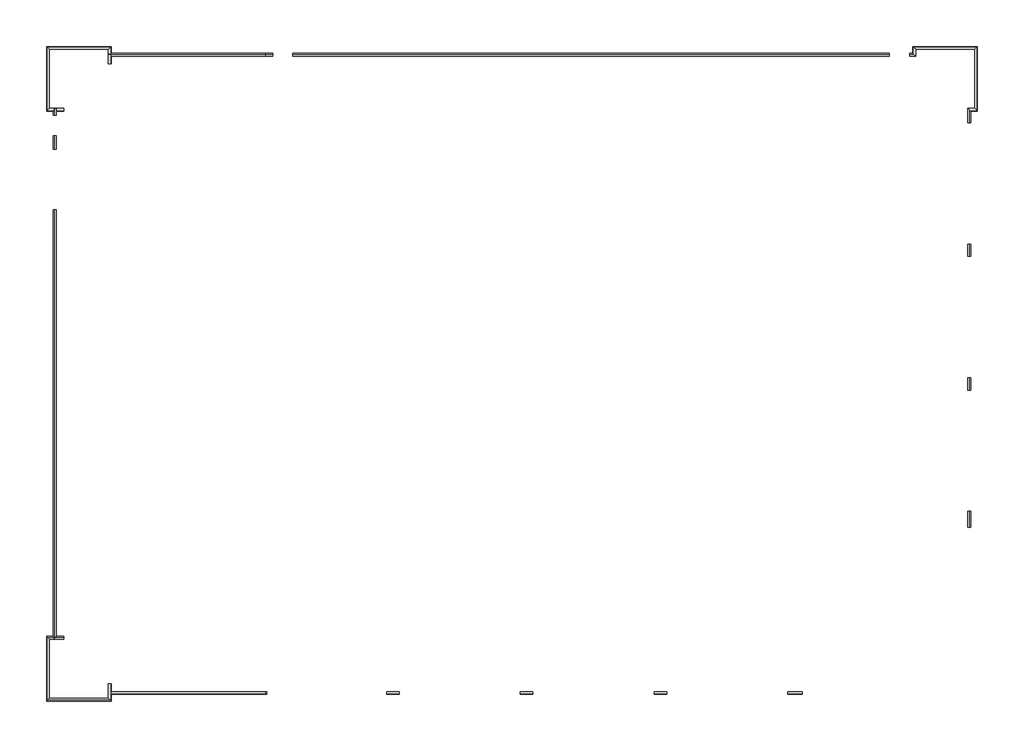
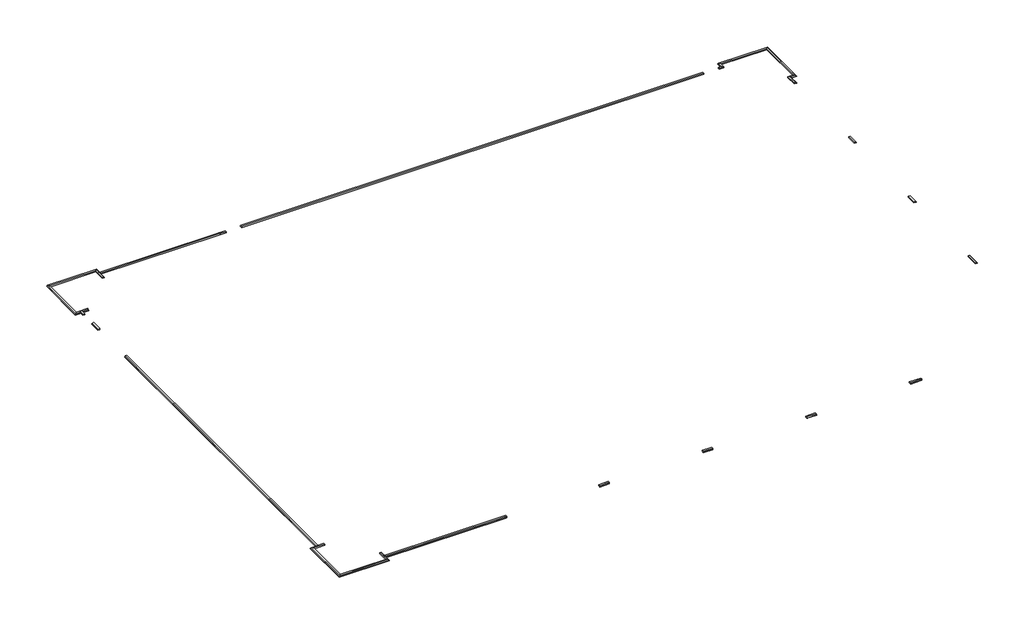
# One storey: 18 proxies.
"""IFC4 building model written with IfcOpenShell, lengths in millimetres."""

from ifc_helpers import new_model, si_unit, origin, place, context, project, spatial, faceted_brep, element, save

model = new_model("IFC4")

# Units and contexts
model_context = context("Model", 3, world=origin())
ifc_project = project(units=[si_unit("LENGTHUNIT", "METRE", prefix="MILLI")], contexts=[model_context])

# Site, building, storey
site = spatial("IfcSite", under=ifc_project)
building = spatial("IfcBuilding", under=site)
storey = spatial("IfcBuildingStorey", under=building, Name="CMU Watertable", Elevation=914.4)

# Proxies
placement = place(None, origin())
element("IfcBuildingElementProxy", 1, Name="Wall Sweeps", at=placement, inside=storey, context=model_context, shape_type="Brep", body=[
    faceted_brep([(-20031.8727721, 14336.3436943, 984.25), (-20031.8727721, 14428.4186943, 984.25), (-20031.8727721, 14463.3436943, 939.8), (-20031.8727721, 14463.3436943, 914.4), (-20031.8727721, 14447.4686943, 914.4), (-20031.8727721, 14336.3436943, 914.4), (-12953.2102721, 14336.3436943, 984.25), (-12953.2102721, 14336.3436943, 914.4), (-12953.2102721, 14345.8686943, 914.4), (-12953.2102721, 14447.4686943, 914.4), (-12953.2102721, 14463.3436943, 914.4), (-12953.2102721, 14463.3436943, 939.8), (-12953.2102721, 14428.4186943, 984.25)], [[[0, 1, 2, 3, 4, 5]], [[6, 7, 8, 9, 10, 11, 12]], [[1, 0, 6, 12]], [[2, 1, 12, 11]], [[3, 2, 11, 10]], [[5, 4, 3, 10, 9, 8, 7]], [[0, 5, 7, 6]]]),
])
element("IfcBuildingElementProxy", 2, Name="Wall Sweeps", at=placement, inside=storey, context=model_context, shape_type="Brep", body=[
    faceted_brep([(18820.6022279, 11967.7936943, 984.25), (18912.6772279, 11875.7186943, 984.25), (18947.6022279, 11840.7936943, 939.8), (18947.6022279, 11840.7936943, 914.4), (18820.6022279, 11967.7936943, 914.4), (18820.6022279, 11321.6811943, 984.25), (18820.6022279, 11321.6811943, 914.4), (18931.7272279, 11321.6811943, 914.4), (18947.6022279, 11321.6811943, 914.4), (18947.6022279, 11321.6811943, 939.8), (18912.6772279, 11321.6811943, 984.25)], [[[0, 1, 2, 3, 4]], [[5, 6, 7, 8, 9, 10]], [[1, 0, 5, 10]], [[2, 1, 10, 9]], [[3, 2, 9, 8]], [[4, 3, 8, 7, 6]], [[0, 4, 6, 5]]]),
    faceted_brep([(18820.6022279, 5835.2811943, 984.25), (18912.6772279, 5835.2811943, 984.25), (18947.6022279, 5835.2811943, 939.8), (18947.6022279, 5835.2811943, 914.4), (18931.7272279, 5835.2811943, 914.4), (18820.6022279, 5835.2811943, 914.4), (18820.6022279, 5276.4811943, 984.25), (18820.6022279, 5276.4811943, 914.4), (18931.7272279, 5276.4811943, 914.4), (18947.6022279, 5276.4811943, 914.4), (18947.6022279, 5276.4811943, 939.8), (18912.6772279, 5276.4811943, 984.25)], [[[0, 1, 2, 3, 4, 5]], [[6, 7, 8, 9, 10, 11]], [[1, 0, 6, 11]], [[2, 1, 11, 10]], [[3, 2, 10, 9]], [[5, 4, 3, 9, 8, 7]], [[0, 5, 7, 6]]]),
    faceted_brep([(18820.6022279, -209.9188057, 984.25), (18912.6772279, -209.9188057, 984.25), (18947.6022279, -209.9188057, 939.8), (18947.6022279, -209.9188057, 914.4), (18931.7272279, -209.9188057, 914.4), (18820.6022279, -209.9188057, 914.4), (18820.6022279, -768.7188057, 984.25), (18820.6022279, -768.7188057, 914.4), (18931.7272279, -768.7188057, 914.4), (18947.6022279, -768.7188057, 914.4), (18947.6022279, -768.7188057, 939.8), (18912.6772279, -768.7188057, 984.25)], [[[0, 1, 2, 3, 4, 5]], [[6, 7, 8, 9, 10, 11]], [[1, 0, 6, 11]], [[2, 1, 11, 10]], [[3, 2, 10, 9]], [[5, 4, 3, 9, 8, 7]], [[0, 5, 7, 6]]]),
    faceted_brep([(18820.6022279, -6255.1188057, 984.25), (18912.6772279, -6255.1188057, 984.25), (18947.6022279, -6255.1188057, 939.8), (18947.6022279, -6255.1188057, 914.4), (18931.7272279, -6255.1188057, 914.4), (18820.6022279, -6255.1188057, 914.4), (18820.6022279, -6969.1417889, 984.25), (18820.6022279, -6969.1417889, 914.4), (18931.7272279, -6969.1417889, 914.4), (18947.6022279, -6969.1417889, 914.4), (18947.6022279, -6969.1417889, 939.8), (18912.6772279, -6969.1417889, 984.25)], [[[0, 1, 2, 3, 4, 5]], [[6, 7, 8, 9, 10, 11]], [[1, 0, 6, 11]], [[2, 1, 11, 10]], [[3, 2, 10, 9]], [[5, 4, 3, 9, 8, 7]], [[0, 5, 7, 6]]]),
])
element("IfcBuildingElementProxy", 3, Name="Wall Sweeps", at=placement, inside=storey, context=model_context, shape_type="Brep", body=[
    faceted_brep([(11340.2095287, -14397.4063057, 984.25), (11340.2095287, -14489.4813057, 984.25), (11340.2095287, -14524.4063057, 939.8), (11340.2095287, -14524.4063057, 914.4), (11340.2095287, -14508.5313057, 914.4), (11340.2095287, -14397.4063057, 914.4), (10678.3147279, -14397.4063057, 984.25), (10678.3147279, -14397.4063057, 914.4), (10678.3147279, -14508.5313057, 914.4), (10678.3147279, -14524.4063057, 914.4), (10678.3147279, -14524.4063057, 939.8), (10678.3147279, -14489.4813057, 984.25)], [[[0, 1, 2, 3, 4, 5]], [[6, 7, 8, 9, 10, 11]], [[1, 0, 6, 11]], [[2, 1, 11, 10]], [[3, 2, 10, 9]], [[5, 4, 3, 9, 8, 7]], [[0, 5, 7, 6]]]),
    faceted_brep([(5191.9147279, -14397.4063057, 984.25), (5191.9147279, -14489.4813057, 984.25), (5191.9147279, -14524.4063057, 939.8), (5191.9147279, -14524.4063057, 914.4), (5191.9147279, -14508.5313057, 914.4), (5191.9147279, -14397.4063057, 914.4), (4633.1147279, -14397.4063057, 984.25), (4633.1147279, -14397.4063057, 914.4), (4633.1147279, -14508.5313057, 914.4), (4633.1147279, -14524.4063057, 914.4), (4633.1147279, -14524.4063057, 939.8), (4633.1147279, -14489.4813057, 984.25)], [[[0, 1, 2, 3, 4, 5]], [[6, 7, 8, 9, 10, 11]], [[1, 0, 6, 11]], [[2, 1, 11, 10]], [[3, 2, 10, 9]], [[5, 4, 3, 9, 8, 7]], [[0, 5, 7, 6]]]),
    faceted_brep([(-853.2852721, -14397.4063057, 984.25), (-853.2852721, -14489.4813057, 984.25), (-853.2852721, -14524.4063057, 939.8), (-853.2852721, -14524.4063057, 914.4), (-853.2852721, -14508.5313057, 914.4), (-853.2852721, -14397.4063057, 914.4), (-1412.0852721, -14397.4063057, 984.25), (-1412.0852721, -14397.4063057, 914.4), (-1412.0852721, -14508.5313057, 914.4), (-1412.0852721, -14524.4063057, 914.4), (-1412.0852721, -14524.4063057, 939.8), (-1412.0852721, -14489.4813057, 984.25)], [[[0, 1, 2, 3, 4, 5]], [[6, 7, 8, 9, 10, 11]], [[1, 0, 6, 11]], [[2, 1, 11, 10]], [[3, 2, 10, 9]], [[5, 4, 3, 9, 8, 7]], [[0, 5, 7, 6]]]),
    faceted_brep([(-6898.4852721, -14397.4063057, 984.25), (-6898.4852721, -14489.4813057, 984.25), (-6898.4852721, -14524.4063057, 939.8), (-6898.4852721, -14524.4063057, 914.4), (-6898.4852721, -14508.5313057, 914.4), (-6898.4852721, -14397.4063057, 914.4), (-7457.2852721, -14397.4063057, 984.25), (-7457.2852721, -14397.4063057, 914.4), (-7457.2852721, -14508.5313057, 914.4), (-7457.2852721, -14524.4063057, 914.4), (-7457.2852721, -14524.4063057, 939.8), (-7457.2852721, -14489.4813057, 984.25)], [[[0, 1, 2, 3, 4, 5]], [[6, 7, 8, 9, 10, 11]], [[1, 0, 6, 11]], [[2, 1, 11, 10]], [[3, 2, 10, 9]], [[5, 4, 3, 9, 8, 7]], [[0, 5, 7, 6]]]),
    faceted_brep([(-12883.3602721, -14397.4063057, 984.25), (-12883.3602721, -14489.4813057, 984.25), (-12883.3602721, -14524.4063057, 939.8), (-12883.3602721, -14524.4063057, 914.4), (-12883.3602721, -14508.5313057, 914.4), (-12883.3602721, -14397.4063057, 914.4), (-12953.2102721, -14397.4063057, 984.25), (-12953.2102721, -14397.4063057, 914.4), (-12953.2102721, -14406.9313057, 914.4), (-12953.2102721, -14508.5313057, 914.4), (-12953.2102721, -14524.4063057, 914.4), (-12953.2102721, -14524.4063057, 939.8), (-12953.2102721, -14489.4813057, 984.25)], [[[0, 1, 2, 3, 4, 5]], [[6, 7, 8, 9, 10, 11, 12]], [[1, 0, 6, 12]], [[2, 1, 12, 11]], [[3, 2, 11, 10]], [[5, 4, 3, 10, 9, 8, 7]], [[0, 5, 7, 6]]]),
])
element("IfcBuildingElementProxy", 4, Name="Wall Sweeps", at=placement, inside=storey, context=model_context, shape_type="Brep", body=[
    faceted_brep([(-22409.9477721, -12019.3313057, 984.25), (-22502.0227721, -12019.3313057, 984.25), (-22536.9477721, -12019.3313057, 939.8), (-22536.9477721, -12019.3313057, 914.4), (-22521.0727721, -12019.3313057, 914.4), (-22409.9477721, -12019.3313057, 914.4), (-22409.9477721, 7386.2686943, 984.25), (-22409.9477721, 7386.2686943, 914.4), (-22521.0727721, 7386.2686943, 914.4), (-22536.9477721, 7386.2686943, 914.4), (-22536.9477721, 7386.2686943, 939.8), (-22502.0227721, 7386.2686943, 984.25)], [[[0, 1, 2, 3, 4, 5]], [[6, 7, 8, 9, 10, 11]], [[1, 0, 6, 11]], [[2, 1, 11, 10]], [[3, 2, 10, 9]], [[5, 4, 3, 9, 8, 7]], [[0, 5, 7, 6]]]),
    faceted_brep([(-22409.9477721, 10129.4686943, 984.25), (-22502.0227721, 10129.4686943, 984.25), (-22536.9477721, 10129.4686943, 939.8), (-22536.9477721, 10129.4686943, 914.4), (-22521.0727721, 10129.4686943, 914.4), (-22409.9477721, 10129.4686943, 914.4), (-22409.9477721, 10739.0686943, 984.25), (-22409.9477721, 10739.0686943, 914.4), (-22521.0727721, 10739.0686943, 914.4), (-22536.9477721, 10739.0686943, 914.4), (-22536.9477721, 10739.0686943, 939.8), (-22502.0227721, 10739.0686943, 984.25)], [[[0, 1, 2, 3, 4, 5]], [[6, 7, 8, 9, 10, 11]], [[1, 0, 6, 11]], [[2, 1, 11, 10]], [[3, 2, 10, 9]], [[5, 4, 3, 9, 8, 7]], [[0, 5, 7, 6]]]),
    faceted_brep([(-22409.9477721, 11653.4686943, 984.25), (-22502.0227721, 11653.4686943, 984.25), (-22536.9477721, 11653.4686943, 939.8), (-22536.9477721, 11653.4686943, 914.4), (-22521.0727721, 11653.4686943, 914.4), (-22409.9477721, 11653.4686943, 914.4), (-22409.9477721, 11958.2686943, 984.25), (-22409.9477721, 11958.2686943, 914.4), (-22521.0727721, 11958.2686943, 914.4), (-22536.9477721, 11958.2686943, 914.4), (-22536.9477721, 11958.2686943, 939.8), (-22502.0227721, 11958.2686943, 984.25)], [[[0, 1, 2, 3, 4, 5]], [[6, 7, 8, 9, 10, 11]], [[1, 0, 6, 11]], [[2, 1, 11, 10]], [[3, 2, 10, 9]], [[5, 4, 3, 9, 8, 7]], [[0, 5, 7, 6]]]),
])
element("IfcBuildingElementProxy", 5, Name="Wall Sweeps", at=placement, inside=storey, context=model_context, shape_type="Brep", body=[
    faceted_brep([(-12953.2102721, 14336.3436943, 984.25), (-12953.2102721, 14428.4186943, 984.25), (-12953.2102721, 14463.3436943, 939.8), (-12953.2102721, 14463.3436943, 914.4), (-12953.2102721, 14447.4686943, 914.4), (-12953.2102721, 14345.8686943, 914.4), (-12953.2102721, 14336.3436943, 914.4), (-12615.0727721, 14336.3436943, 984.25), (-12615.0727721, 14336.3436943, 914.4), (-12615.0727721, 14447.4686943, 914.4), (-12615.0727721, 14463.3436943, 914.4), (-12615.0727721, 14463.3436943, 939.8), (-12615.0727721, 14428.4186943, 984.25)], [[[0, 1, 2, 3, 4, 5, 6]], [[7, 8, 9, 10, 11, 12]], [[1, 0, 7, 12]], [[2, 1, 12, 11]], [[3, 2, 11, 10]], [[6, 5, 4, 3, 10, 9, 8]], [[0, 6, 8, 7]]]),
    faceted_brep([(-11700.6727721, 14336.3436943, 984.25), (-11700.6727721, 14428.4186943, 984.25), (-11700.6727721, 14463.3436943, 939.8), (-11700.6727721, 14463.3436943, 914.4), (-11700.6727721, 14447.4686943, 914.4), (-11700.6727721, 14336.3436943, 914.4), (15274.1272279, 14336.3436943, 984.25), (15274.1272279, 14336.3436943, 914.4), (15274.1272279, 14447.4686943, 914.4), (15274.1272279, 14463.3436943, 914.4), (15274.1272279, 14463.3436943, 939.8), (15274.1272279, 14428.4186943, 984.25)], [[[0, 1, 2, 3, 4, 5]], [[6, 7, 8, 9, 10, 11]], [[1, 0, 6, 11]], [[2, 1, 11, 10]], [[3, 2, 10, 9]], [[5, 4, 3, 9, 8, 7]], [[0, 5, 7, 6]]]),
    faceted_brep([(16188.5272279, 14336.3436943, 984.25), (16188.5272279, 14428.4186943, 984.25), (16188.5272279, 14463.3436943, 939.8), (16188.5272279, 14463.3436943, 914.4), (16188.5272279, 14447.4686943, 914.4), (16188.5272279, 14336.3436943, 914.4), (16452.0522279, 14336.3436943, 984.25), (16452.0522279, 14336.3436943, 914.4), (16325.0522279, 14463.3436943, 914.4), (16325.0522279, 14463.3436943, 939.8), (16359.9772279, 14428.4186943, 984.25)], [[[0, 1, 2, 3, 4, 5]], [[6, 7, 8, 9, 10]], [[1, 0, 6, 10]], [[2, 1, 10, 9]], [[3, 2, 9, 8]], [[5, 4, 3, 8, 7]], [[0, 5, 7, 6]]]),
])
element("IfcBuildingElementProxy", 6, Name="Wall Sweeps", at=placement, inside=storey, context=model_context, shape_type="Brep", body=[
    faceted_brep([(-12953.2102721, -14397.4063057, 984.25), (-12953.2102721, -14489.4813057, 984.25), (-12953.2102721, -14524.4063057, 939.8), (-12953.2102721, -14524.4063057, 914.4), (-12953.2102721, -14508.5313057, 914.4), (-12953.2102721, -14406.9313057, 914.4), (-12953.2102721, -14397.4063057, 914.4), (-20031.8727721, -14397.4063057, 984.25), (-20031.8727721, -14397.4063057, 914.4), (-20031.8727721, -14508.5313057, 914.4), (-20031.8727721, -14524.4063057, 914.4), (-20031.8727721, -14524.4063057, 939.8), (-20031.8727721, -14489.4813057, 984.25)], [[[0, 1, 2, 3, 4, 5, 6]], [[7, 8, 9, 10, 11, 12]], [[1, 0, 7, 12]], [[2, 1, 12, 11]], [[3, 2, 11, 10]], [[6, 5, 4, 3, 10, 9, 8]], [[0, 6, 8, 7]]]),
])
element("IfcBuildingElementProxy", 7, Name="Wall Sweeps", at=placement, inside=storey, context=model_context, shape_type="Brep", body=[
    faceted_brep([(-20041.3977721, 13993.4436943, 984.25), (-20041.3977721, 13993.4436943, 914.4), (-19930.2727721, 13993.4436943, 914.4), (-19914.3977721, 13993.4436943, 914.4), (-19914.3977721, 13993.4436943, 939.8), (-19949.3227721, 13993.4436943, 984.25), (-20041.3977721, 14641.1436943, 984.25), (-19949.3227721, 14733.2186943, 984.25), (-19914.3977721, 14768.1436943, 939.8), (-19914.3977721, 14768.1436943, 914.4), (-20041.3977721, 14641.1436943, 914.4)], [[[0, 1, 2, 3, 4, 5]], [[6, 7, 8, 9, 10]], [[1, 0, 6, 10]], [[3, 2, 1, 10, 9]], [[4, 3, 9, 8]], [[5, 4, 8, 7]], [[0, 5, 7, 6]]]),
])
element("IfcBuildingElementProxy", 8, Name="Wall Sweeps", at=placement, inside=storey, context=model_context, shape_type="Brep", body=[
    faceted_brep([(-20041.3977721, 14641.1436943, 984.25), (-20041.3977721, 14641.1436943, 914.4), (-19914.3977721, 14768.1436943, 914.4), (-19914.3977721, 14768.1436943, 939.8), (-19949.3227721, 14733.2186943, 984.25), (-22714.7477721, 14641.1436943, 984.25), (-22806.8227721, 14733.2186943, 984.25), (-22841.7477721, 14768.1436943, 939.8), (-22841.7477721, 14768.1436943, 914.4), (-22714.7477721, 14641.1436943, 914.4)], [[[0, 1, 2, 3, 4]], [[5, 6, 7, 8, 9]], [[1, 0, 5, 9]], [[2, 1, 9, 8]], [[3, 2, 8, 7]], [[4, 3, 7, 6]], [[0, 4, 6, 5]]]),
])
element("IfcBuildingElementProxy", 9, Name="Wall Sweeps", at=placement, inside=storey, context=model_context, shape_type="Brep", body=[
    faceted_brep([(-22714.7477721, 14641.1436943, 984.25), (-22714.7477721, 14641.1436943, 914.4), (-22841.7477721, 14768.1436943, 914.4), (-22841.7477721, 14768.1436943, 939.8), (-22806.8227721, 14733.2186943, 984.25), (-22714.7477721, 11967.7936943, 984.25), (-22806.8227721, 11875.7186943, 984.25), (-22841.7477721, 11840.7936943, 939.8), (-22841.7477721, 11840.7936943, 914.4), (-22714.7477721, 11967.7936943, 914.4)], [[[0, 1, 2, 3, 4]], [[5, 6, 7, 8, 9]], [[1, 0, 5, 9]], [[2, 1, 9, 8]], [[3, 2, 8, 7]], [[4, 3, 7, 6]], [[0, 4, 6, 5]]]),
])
element("IfcBuildingElementProxy", 10, Name="Wall Sweeps", at=placement, inside=storey, context=model_context, shape_type="Brep", body=[
    faceted_brep([(-22714.7477721, 11967.7936943, 984.25), (-22714.7477721, 11967.7936943, 914.4), (-22841.7477721, 11840.7936943, 914.4), (-22841.7477721, 11840.7936943, 939.8), (-22806.8227721, 11875.7186943, 984.25), (-22067.0477721, 11967.7936943, 984.25), (-22067.0477721, 11875.7186943, 984.25), (-22067.0477721, 11840.7936943, 939.8), (-22067.0477721, 11840.7936943, 914.4), (-22067.0477721, 11856.6686943, 914.4), (-22067.0477721, 11967.7936943, 914.4)], [[[0, 1, 2, 3, 4]], [[5, 6, 7, 8, 9, 10]], [[1, 0, 5, 10]], [[2, 1, 10, 9, 8]], [[3, 2, 8, 7]], [[4, 3, 7, 6]], [[0, 4, 6, 5]]]),
])
element("IfcBuildingElementProxy", 11, Name="Wall Sweeps", at=placement, inside=storey, context=model_context, shape_type="Brep", body=[
    faceted_brep([(-20041.3977721, -14054.5063057, 984.25), (-19949.3227721, -14054.5063057, 984.25), (-19914.3977721, -14054.5063057, 939.8), (-19914.3977721, -14054.5063057, 914.4), (-19930.2727721, -14054.5063057, 914.4), (-20041.3977721, -14054.5063057, 914.4), (-20041.3977721, -14702.2063057, 984.25), (-20041.3977721, -14702.2063057, 914.4), (-19914.3977721, -14829.2063057, 914.4), (-19914.3977721, -14829.2063057, 939.8), (-19949.3227721, -14794.2813057, 984.25)], [[[0, 1, 2, 3, 4, 5]], [[6, 7, 8, 9, 10]], [[1, 0, 6, 10]], [[2, 1, 10, 9]], [[3, 2, 9, 8]], [[5, 4, 3, 8, 7]], [[0, 5, 7, 6]]]),
])
element("IfcBuildingElementProxy", 12, Name="Wall Sweeps", at=placement, inside=storey, context=model_context, shape_type="Brep", body=[
    faceted_brep([(-20041.3977721, -14702.2063057, 984.25), (-19949.3227721, -14794.2813057, 984.25), (-19914.3977721, -14829.2063057, 939.8), (-19914.3977721, -14829.2063057, 914.4), (-20041.3977721, -14702.2063057, 914.4), (-22714.7477721, -14702.2063057, 984.25), (-22714.7477721, -14702.2063057, 914.4), (-22841.7477721, -14829.2063057, 914.4), (-22841.7477721, -14829.2063057, 939.8), (-22806.8227721, -14794.2813057, 984.25)], [[[0, 1, 2, 3, 4]], [[5, 6, 7, 8, 9]], [[1, 0, 5, 9]], [[2, 1, 9, 8]], [[3, 2, 8, 7]], [[4, 3, 7, 6]], [[0, 4, 6, 5]]]),
])
element("IfcBuildingElementProxy", 13, Name="Wall Sweeps", at=placement, inside=storey, context=model_context, shape_type="Brep", body=[
    faceted_brep([(-22714.7477721, -14702.2063057, 984.25), (-22806.8227721, -14794.2813057, 984.25), (-22841.7477721, -14829.2063057, 939.8), (-22841.7477721, -14829.2063057, 914.4), (-22714.7477721, -14702.2063057, 914.4), (-22714.7477721, -12028.8563057, 984.25), (-22714.7477721, -12028.8563057, 914.4), (-22841.7477721, -11901.8563057, 914.4), (-22841.7477721, -11901.8563057, 939.8), (-22806.8227721, -11936.7813057, 984.25)], [[[0, 1, 2, 3, 4]], [[5, 6, 7, 8, 9]], [[1, 0, 5, 9]], [[2, 1, 9, 8]], [[3, 2, 8, 7]], [[4, 3, 7, 6]], [[0, 4, 6, 5]]]),
])
element("IfcBuildingElementProxy", 14, Name="Wall Sweeps", at=placement, inside=storey, context=model_context, shape_type="Brep", body=[
    faceted_brep([(-22714.7477721, -12028.8563057, 984.25), (-22806.8227721, -11936.7813057, 984.25), (-22841.7477721, -11901.8563057, 939.8), (-22841.7477721, -11901.8563057, 914.4), (-22714.7477721, -12028.8563057, 914.4), (-22067.0477721, -12028.8563057, 984.25), (-22067.0477721, -12028.8563057, 914.4), (-22067.0477721, -11917.7313057, 914.4), (-22067.0477721, -11901.8563057, 914.4), (-22067.0477721, -11901.8563057, 939.8), (-22067.0477721, -11936.7813057, 984.25)], [[[0, 1, 2, 3, 4]], [[5, 6, 7, 8, 9, 10]], [[1, 0, 5, 10]], [[2, 1, 10, 9]], [[3, 2, 9, 8]], [[4, 3, 8, 7, 6]], [[0, 4, 6, 5]]]),
])
element("IfcBuildingElementProxy", 15, Name="Wall Sweeps", at=placement, inside=storey, context=model_context, shape_type="Brep", body=[
    faceted_brep([(16452.0522279, 14336.3436943, 984.25), (16359.9772279, 14428.4186943, 984.25), (16325.0522279, 14463.3436943, 939.8), (16325.0522279, 14463.3436943, 914.4), (16452.0522279, 14336.3436943, 914.4), (16452.0522279, 14641.1436943, 984.25), (16452.0522279, 14641.1436943, 914.4), (16325.0522279, 14768.1436943, 914.4), (16325.0522279, 14768.1436943, 939.8), (16359.9772279, 14733.2186943, 984.25)], [[[0, 1, 2, 3, 4]], [[5, 6, 7, 8, 9]], [[1, 0, 5, 9]], [[2, 1, 9, 8]], [[3, 2, 8, 7]], [[4, 3, 7, 6]], [[0, 4, 6, 5]]]),
])
element("IfcBuildingElementProxy", 16, Name="Wall Sweeps", at=placement, inside=storey, context=model_context, shape_type="Brep", body=[
    faceted_brep([(16452.0522279, 14641.1436943, 984.25), (16359.9772279, 14733.2186943, 984.25), (16325.0522279, 14768.1436943, 939.8), (16325.0522279, 14768.1436943, 914.4), (16452.0522279, 14641.1436943, 914.4), (19125.4022279, 14641.1436943, 984.25), (19125.4022279, 14641.1436943, 914.4), (19252.4022279, 14768.1436943, 914.4), (19252.4022279, 14768.1436943, 939.8), (19217.4772279, 14733.2186943, 984.25)], [[[0, 1, 2, 3, 4]], [[5, 6, 7, 8, 9]], [[1, 0, 5, 9]], [[2, 1, 9, 8]], [[3, 2, 8, 7]], [[4, 3, 7, 6]], [[0, 4, 6, 5]]]),
])
element("IfcBuildingElementProxy", 17, Name="Wall Sweeps", at=placement, inside=storey, context=model_context, shape_type="Brep", body=[
    faceted_brep([(19125.4022279, 14641.1436943, 984.25), (19217.4772279, 14733.2186943, 984.25), (19252.4022279, 14768.1436943, 939.8), (19252.4022279, 14768.1436943, 914.4), (19125.4022279, 14641.1436943, 914.4), (19125.4022279, 11967.7936943, 984.25), (19125.4022279, 11967.7936943, 914.4), (19252.4022279, 11840.7936943, 914.4), (19252.4022279, 11840.7936943, 939.8), (19217.4772279, 11875.7186943, 984.25)], [[[0, 1, 2, 3, 4]], [[5, 6, 7, 8, 9]], [[1, 0, 5, 9]], [[2, 1, 9, 8]], [[3, 2, 8, 7]], [[4, 3, 7, 6]], [[0, 4, 6, 5]]]),
])
element("IfcBuildingElementProxy", 18, Name="Wall Sweeps", at=placement, inside=storey, context=model_context, shape_type="Brep", body=[
    faceted_brep([(19125.4022279, 11967.7936943, 984.25), (19217.4772279, 11875.7186943, 984.25), (19252.4022279, 11840.7936943, 939.8), (19252.4022279, 11840.7936943, 914.4), (19125.4022279, 11967.7936943, 914.4), (18820.6022279, 11967.7936943, 984.25), (18820.6022279, 11967.7936943, 914.4), (18947.6022279, 11840.7936943, 914.4), (18947.6022279, 11840.7936943, 939.8), (18912.6772279, 11875.7186943, 984.25)], [[[0, 1, 2, 3, 4]], [[5, 6, 7, 8, 9]], [[1, 0, 5, 9]], [[2, 1, 9, 8]], [[3, 2, 8, 7]], [[4, 3, 7, 6]], [[0, 4, 6, 5]]]),
])

save(model, "model.ifc")

# Revit data of these elements
# Project information
#   Project Issue Date = "Issue Date"
#   Project Status = "Project Status"
#   Client Name = "Owner"
#   Project Address = "Enter address here"
#   Project Name = "Pharmacy"
#   Project Number = "Project Number"
# Grids (mm)
#   "1": line (-22521.073, -18946.14) -> (-22521.073, 18514.621)
#   "2": line (-12943.685, 18514.621) -> (-12943.685, -18946.14)
#   "4": line (4937.915, 18514.621) -> (4937.915, -18946.14)
#   "5": line (13154.021, 18514.621) -> (13154.021, -18946.14)
#   "6": line (18931.727, 18514.621) -> (18931.727, -18946.14)
#   "6.5": line (21370.127, 18514.621) -> (21370.127, -18946.14)
#   "A": line (-28029.004, 14447.469) -> (24344.828, 14447.469)
#   "C": line (-28029.004, -514.719) -> (24344.828, -514.719)
#   "D": line (-28029.004, -8730.825) -> (24344.828, -8730.825)
#   "E": line (-28029.004, -14508.531) -> (24344.828, -14508.531)
#   "E.5": line (-28029.004, -16946.931) -> (24344.828, -16946.931)
#   "3": line (-7177.885, 18514.621) -> (-7177.885, -18946.14)
#   "B": line (-28029.004, 5555.881) -> (24344.828, 5555.881)
# Elements 1, 2, 3, 4, 5, 6, 7, 8, 9, 10, 11, 12, 13, 14, 15, 16, 17, 18 (IfcBuildingElementProxy)
#   Phase Created = New Construction
#   Materials on its faces: "Concrete - Cast-in-Place Concrete"
# Materials
#   "Concrete - Cast-in-Place Concrete": class "Concrete", colour RGB 192 192 192, transparency 0, Cost = 0
